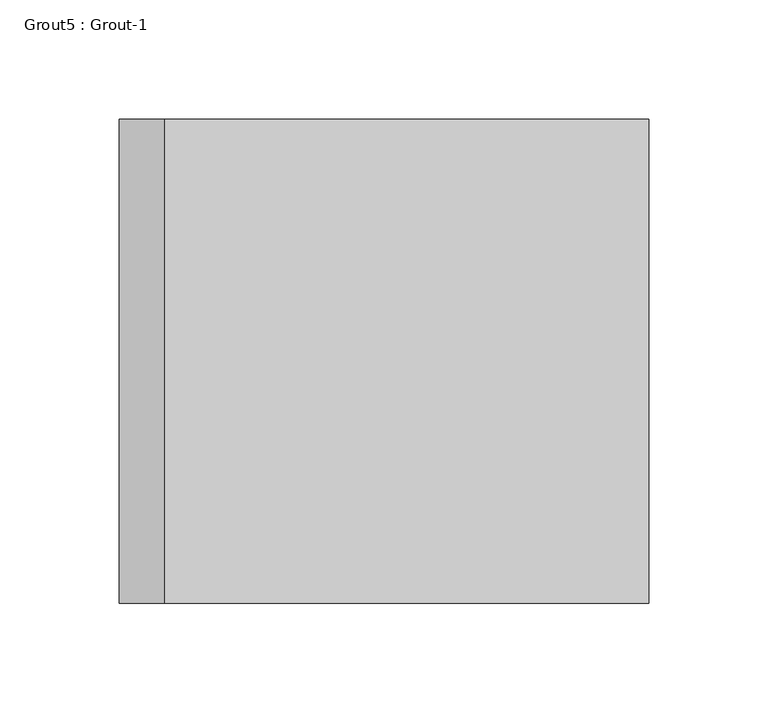
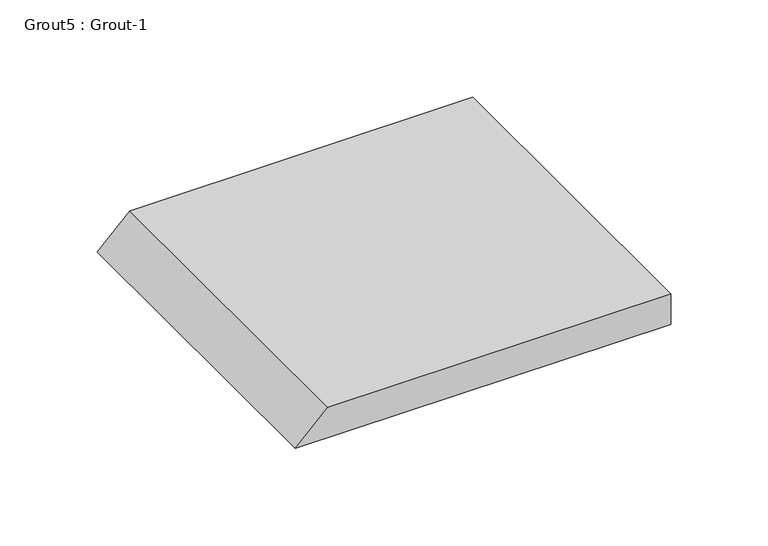
"""IFC4 building model written with IfcOpenShell, lengths in millimetres: proxy geometry, Grout5 : Grout-1."""

import ifcopenshell
import ifcopenshell.guid

model = None  # the IFC model being written
_history = None  # IfcOwnerHistory: only IFC2X3 demands one
_inside = {}  # id of a spatial element -> (the spatial element, [elements in it])
_under = {}  # id of a project, library or spatial element -> (it, [spatial elements below it])
_declared = {}  # id of a project -> (the project, [libraries it declares])
_typed = {}  # id of a type object -> (the type object, [elements of that type])
_made_of = {}  # id of a material, layer set ... -> (it, [elements and type objects made of it])


def new_model(schema):
    """Start an empty IFC model of exactly this schema.

    Asked for "IFC4X3", IfcOpenShell would pick the latest addendum, in which some entities
    have other attributes; the version numbers below select the first issue.
    IFC2X3 requires an IfcOwnerHistory on every rooted entity: one is made here for all.
    """
    global model, _history
    if schema == "IFC4X3":
        model = ifcopenshell.file(schema_version=(4, 3, 0, 0))
    else:
        model = ifcopenshell.file(schema=schema)
    _inside.clear()
    _under.clear()
    _declared.clear()
    _typed.clear()
    _made_of.clear()
    _history = None
    if model.schema == "IFC2X3":
        org = make("IfcOrganization", Name="unknown")
        user = make(
            "IfcPersonAndOrganization",
            ThePerson=make("IfcPerson", FamilyName="unknown"),
            TheOrganization=org,
        )
        app = make(
            "IfcApplication",
            ApplicationDeveloper=org,
            Version="unknown",
            ApplicationFullName="unknown",
            ApplicationIdentifier="unknown",
        )
        _history = make(
            "IfcOwnerHistory",
            OwningUser=user,
            OwningApplication=app,
            ChangeAction="ADDED",
            CreationDate=0,
        )
    return model


def make(cls, **values):
    """One entity of the class cls with the attributes given. An attribute that is None is left unset."""
    return model.create_entity(
        cls, **{name: value for name, value in values.items() if value is not None}
    )


def rooted(cls, **values):
    """An entity with a GlobalId (a new one), such as an element, a storey or a relation."""
    return make(cls, GlobalId=ifcopenshell.guid.new(), OwnerHistory=_history, **values)


def si_unit(unit_type, name, prefix=None):
    """IfcSIUnit, for example si_unit("LENGTHUNIT", "METRE", prefix="MILLI")."""
    return make("IfcSIUnit", UnitType=unit_type, Prefix=prefix, Name=name)


def assignment(units):
    """IfcUnitAssignment: the units of a project."""
    return None if units is None else make("IfcUnitAssignment", Units=units)


def point(xyz):
    """IfcCartesianPoint."""
    return None if xyz is None else make("IfcCartesianPoint", Coordinates=xyz)


def direction(xyz):
    """IfcDirection."""
    return None if xyz is None else make("IfcDirection", DirectionRatios=xyz)


def frame(location, z_axis=None, x_axis=None):
    """IfcAxis2Placement3D, a coordinate frame: its origin and axes. An axis left out is left unset."""
    return make(
        "IfcAxis2Placement3D",
        Location=point(location),
        Axis=direction(z_axis),
        RefDirection=direction(x_axis),
    )


def origin():
    """The frame at (0, 0, 0) with its axes left unset."""
    return frame((0.0, 0.0, 0.0))


def place(relative_to, where):
    """IfcLocalPlacement: puts the frame where relative to a parent placement (None: the world)."""
    return make(
        "IfcLocalPlacement", PlacementRelTo=relative_to, RelativePlacement=where
    )


def context(
    kind, dimensions, precision=None, world=None, true_north=None, identifier=None
):
    """IfcGeometricRepresentationContext, for example the 3D "Model" context."""
    return make(
        "IfcGeometricRepresentationContext",
        ContextIdentifier=identifier,
        ContextType=kind,
        CoordinateSpaceDimension=dimensions,
        Precision=precision,
        WorldCoordinateSystem=world,
        TrueNorth=true_north,
    )


def project(units=None, contexts=None):
    """IfcProject with its units and contexts."""
    return rooted(
        "IfcProject",
        Name="project",
        RepresentationContexts=contexts,
        UnitsInContext=assignment(units),
    )


def spatial(cls, under=None, at=None, **own):
    """A site, building, storey or space (cls), placed at a placement, below another one or the project."""
    s = rooted(cls, ObjectPlacement=at, **own)
    if under is not None:
        _under.setdefault(under.id(), (under, []))[1].append(s)
    return s


def polyline(points):
    """IfcPolyline through the points."""
    return make("IfcPolyline", Points=[point(p) for p in points])


def outline(outer, holes=None, kind="AREA"):
    """IfcArbitraryClosedProfileDef: a profile drawn as a closed curve; with holes, ...WithVoids."""
    if holes is None:
        return make("IfcArbitraryClosedProfileDef", ProfileType=kind, OuterCurve=outer)
    return make(
        "IfcArbitraryProfileDefWithVoids",
        ProfileType=kind,
        OuterCurve=outer,
        InnerCurves=holes,
    )


def extrude(swept, where, along, depth):
    """IfcExtrudedAreaSolid: the profile swept, set in the frame where, extruded along a direction by depth."""
    return make(
        "IfcExtrudedAreaSolid",
        SweptArea=swept,
        Position=where,
        ExtrudedDirection=direction(along),
        Depth=depth,
    )


def shape(context_of_items, identifier, shape_type, items):
    """IfcShapeRepresentation: the items that make up one representation, for example the "Body"."""
    return make(
        "IfcShapeRepresentation",
        ContextOfItems=context_of_items,
        RepresentationIdentifier=identifier,
        RepresentationType=shape_type,
        Items=items,
    )


def source(mapping_origin, context_of_items, identifier, shape_type, items):
    """IfcRepresentationMap: a shape defined once, which mapped items show again and again."""
    return make(
        "IfcRepresentationMap",
        MappingOrigin=mapping_origin,
        MappedRepresentation=shape(context_of_items, identifier, shape_type, items),
    )


def transform(
    local_origin,
    x_axis=None,
    y_axis=None,
    z_axis=None,
    scale=None,
    scale2=None,
    scale3=None,
    uniform=True,
):
    """IfcCartesianTransformationOperator3D, or its non-uniform kind. x_axis, y_axis, z_axis: its Axis1, 2, 3."""
    if uniform:
        return make(
            "IfcCartesianTransformationOperator3D",
            Axis1=direction(x_axis),
            Axis2=direction(y_axis),
            LocalOrigin=point(local_origin),
            Scale=scale,
            Axis3=direction(z_axis),
        )
    return make(
        "IfcCartesianTransformationOperator3DnonUniform",
        Axis1=direction(x_axis),
        Axis2=direction(y_axis),
        LocalOrigin=point(local_origin),
        Scale=scale,
        Axis3=direction(z_axis),
        Scale2=scale2,
        Scale3=scale3,
    )


def mapped(mapping_source, mapping_target):
    """IfcMappedItem: shows the shape of a source again, moved by a transform."""
    return make(
        "IfcMappedItem", MappingSource=mapping_source, MappingTarget=mapping_target
    )


def made_of(thing, what):
    """Note that an element or type object is made of a material, layer set ...; save() writes the relation."""
    if what is not None:
        _made_of.setdefault(what.id(), (what, []))[1].append(thing)
    return thing


def element(
    cls,
    number,
    at=None,
    inside=None,
    cuts=None,
    type_object=None,
    material=None,
    context=None,
    identifier="Body",
    shape_type=None,
    held_by="IfcProductDefinitionShape",
    body=None,
    shapes=None,
    **own,
):
    """One element of the class cls, such as IfcWall. Its Tag is "e" and its number.

    at: its placement. inside: the storey or other place that contains it. cuts: it is an
    opening in that element (IfcRelVoidsElement). A single representation is given by context,
    identifier, shape_type and body (its items); several are given by shapes. held_by: the class
    of the entity that holds the representations. save() writes the other relations.
    """
    e = rooted(cls, Tag="e%d" % number, ObjectPlacement=at, **own)
    if body is not None:
        shapes = [shape(context, identifier, shape_type, body)]
    if shapes is not None:
        e.Representation = make(held_by, Representations=shapes)
    if inside is not None:
        _inside.setdefault(inside.id(), (inside, []))[1].append(e)
    if cuts is not None:
        rooted(
            "IfcRelVoidsElement", RelatingBuildingElement=cuts, RelatedOpeningElement=e
        )
    if type_object is not None:
        _typed.setdefault(type_object.id(), (type_object, []))[1].append(e)
    return made_of(e, material)


def aggregate(whole, parts):
    """IfcRelAggregates: a whole, such as a stair, and the parts it consists of."""
    return rooted("IfcRelAggregates", RelatingObject=whole, RelatedObjects=parts)


def save(model, path):
    """Write the relations noted so far, then the file.

    IfcRelAggregates (storeys below a building ...), IfcRelContainedInSpatialStructure (elements
    in a storey), IfcRelDefinesByType, IfcRelAssociatesMaterial and IfcRelDeclares: one each for
    every whole, place, type object, material and project.
    """
    for whole, parts in _under.values():
        aggregate(whole, parts)
    for where, things in _inside.values():
        rooted(
            "IfcRelContainedInSpatialStructure",
            RelatedElements=things,
            RelatingStructure=where,
        )
    for kind, things in _typed.values():
        rooted("IfcRelDefinesByType", RelatedObjects=things, RelatingType=kind)
    for what, things in _made_of.values():
        rooted("IfcRelAssociatesMaterial", RelatedObjects=things, RelatingMaterial=what)
    for by, libraries in _declared.values():
        rooted("IfcRelDeclares", RelatingContext=by, RelatedDefinitions=libraries)
    model.write(path)


def grout5_grout_1_e9fd96e3(model_context):
    return source(origin(), model_context, "Body", "SweptSolid", [
        extrude(outline(polyline([(19.05, 590115.4434739), (0.0, 590096.3934739), (0.0, 590318.6434739), (19.05, 590318.6434739), (19.05, 590115.4434739)])), frame((0.0, -534144.2913841, 0.0), z_axis=(0.0, 1.0, 0.0), x_axis=(0.0, 0.0, 1.0)), (0.0, 0.0, 1.0), 203.2),
    ])


if __name__ == "__main__":
    model = new_model("IFC4")
    model_context = context("Model", 3, world=origin())
    ifc_project = project(units=[si_unit("LENGTHUNIT", "METRE", prefix="MILLI")], contexts=[model_context])
    site = spatial("IfcSite", under=ifc_project)
    building = spatial("IfcBuilding", under=site)
    placement = place(None, origin())
    grout5_grout_1_shape = grout5_grout_1_e9fd96e3(model_context)
    element("IfcBuildingElementProxy", 1, Name="Grout5 : Grout-1", ObjectType="Grout5 : Grout-1", at=placement, inside=building, context=model_context, shape_type="MappedRepresentation", body=[
        mapped(grout5_grout_1_shape, transform((0.0, 0.0, 0.0), x_axis=(1.0, 0.0, 0.0), y_axis=(0.0, 1.0, 0.0), z_axis=(0.0, 0.0, 1.0))),
    ])
    save(model, "model.ifc")

# Revit data of these elements
# Element 1 (IfcBuildingElementProxy, "Grout5 : Grout-1")
#   Materials on its faces: "3/4\" NON SHRINK GROUT"
# Materials
#   "3/4\" NON SHRINK GROUT": class "Generic", colour RGB 145 145 143, transparency 0, Cost = 0
